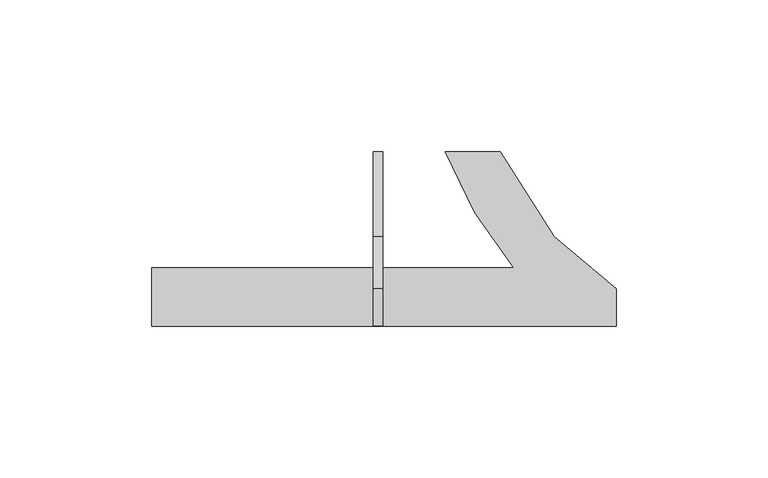
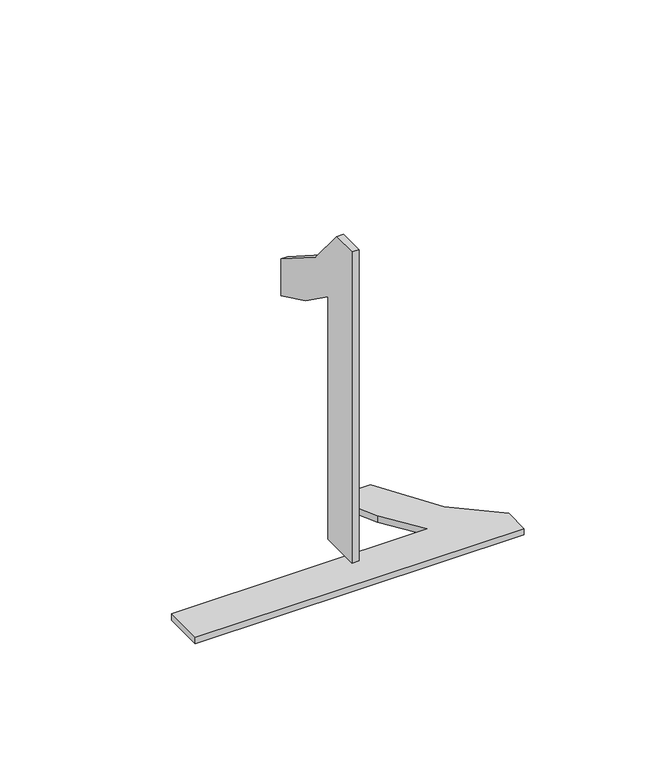
"""IFC4 building model written with IfcOpenShell, lengths in millimetres: proxy geometry, Grid Number2_FedEx : Grid Number2_FedEx."""

from ifc_helpers import new_model, si_unit, frame, origin, origin_with_axes, place, context, project, spatial, polyline, outline, extrude, source, transform, mapped, element, save


def entourage_ecdd8234(model_context):
    return source(origin(), model_context, "Body", "SweptSolid", [
        extrude(outline(polyline([(-184.2739267, 199.7955756), (-184.2739267, 218.9325027), (-64.967147, 218.9325027), (-77.8808351, 237.0602559), (-87.5427406, 257.2063569), (-69.4523642, 257.2063569), (-51.5488719, 229.1550604), (-31.1785101, 212.1299231), (-31.1785101, 199.7955756), (-184.2739267, 199.7955756)])), origin_with_axes(), (0.0, 0.0, 1.0), 3.175),
        extrude(outline(polyline([(199.7955756, 14.2382753), (199.7955756, 167.333692), (212.1299231, 167.333692), (229.1550604, 146.9633301), (257.2063569, 129.0598378), (257.2063569, 110.9694614), (237.0602559, 120.631367), (218.9325027, 133.5450551), (218.9325027, 14.2382753), (199.7955756, 14.2382753)])), frame((-111.2489267, 0.0, 0.0), z_axis=(1.0, 0.0, 0.0), x_axis=(0.0, 1.0, 0.0)), (0.0, 0.0, 1.0), 3.175),
    ])


if __name__ == "__main__":
    model = new_model("IFC4")
    model_context = context("Model", 3, world=origin())
    ifc_project = project(units=[si_unit("LENGTHUNIT", "METRE", prefix="MILLI")], contexts=[model_context])
    site = spatial("IfcSite", under=ifc_project)
    building = spatial("IfcBuilding", under=site)
    placement = place(None, origin())
    entourage_shape = entourage_ecdd8234(model_context)
    element("IfcBuildingElementProxy", 1, Name="Grid Number2_FedEx : Grid Number2_FedEx", ObjectType="Grid Number2_FedEx : Grid Number2_FedEx", at=placement, inside=building, context=model_context, shape_type="MappedRepresentation", body=[
        mapped(entourage_shape, transform((0.0, 0.0, 0.0), x_axis=(1.0, 0.0, 0.0), y_axis=(0.0, 1.0, 0.0), z_axis=(0.0, 0.0, 1.0))),
    ])
    save(model, "model.ifc")

# Revit data of these elements
# Type "Grid Number2_FedEx : Grid Number2_FedEx"
#   Grid [instance default] = "S"
#   Label Width [instance default] = 1' - 0"
#   Half Box Width2 [instance default] = 0' - 6.13846"
#   Half Box Width [instance default] = 0' - 6"
#   Robust [instance default] = yes
#   Height = 0
#   Assembly Code = ""
# Element 1 (IfcBuildingElementProxy, "Grid Number2_FedEx : Grid Number2_FedEx")
#   Grid = "1"
#   Robust = no
#   Materials on its faces: "Letter"
# Materials
#   "Letter": class "Unassigned", colour RGB 178 187 30, transparency 0, Comments = "Rendering appearance not upgraded "
